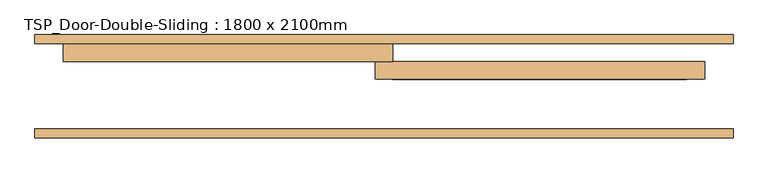
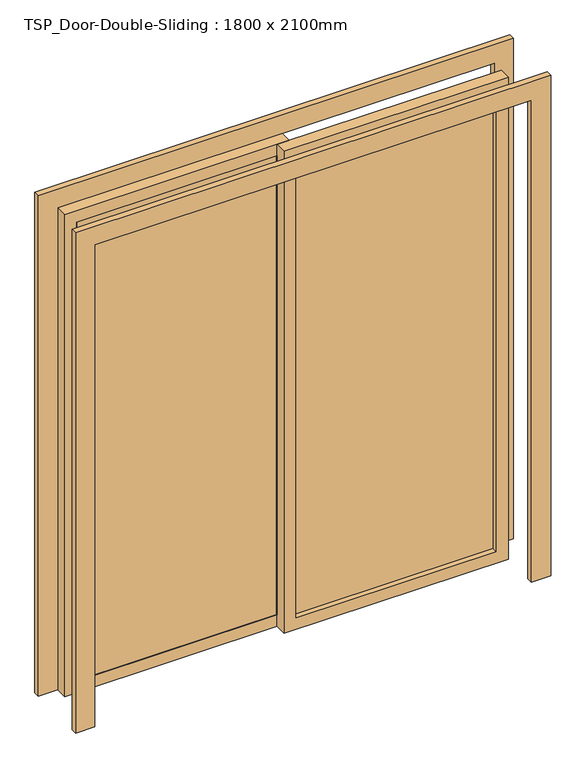
"""IFC4 building model written with IfcOpenShell, lengths in millimetres: door geometry, TSP_Door-Double-Sliding : 1800 x 2100mm."""

from ifc_helpers import new_model, si_unit, frame, origin, place, context, project, spatial, polyline, outline, extrude, source, transform, mapped, element, save


def tsp_door_double_sliding_1800_x_2100mm_5610fb06(model_context):
    return source(origin(), model_context, "Body", "SweptSolid", [
        extrude(outline(polyline([(0.0, 980.0), (2180.0, 980.0), (2180.0, -980.0), (0.0, -980.0), (0.0, -900.0), (2100.0, -900.0), (2100.0, 900.0), (0.0, 900.0), (0.0, 980.0)])), frame((0.0, 247.0, 0.0), z_axis=(0.0, 1.0, 0.0), x_axis=(0.0, 0.0, 1.0)), (0.0, 0.0, 1.0), 25.0),
        extrude(outline(polyline([(0.0, -980.0), (0.0, -900.0), (2100.0, -900.0), (2100.0, 900.0), (0.0, 900.0), (0.0, 980.0), (2180.0, 980.0), (2180.0, -980.0), (0.0, -980.0)])), frame((0.0, -18.0, 0.0), z_axis=(0.0, 1.0, 0.0), x_axis=(0.0, 0.0, 1.0)), (0.0, 0.0, 1.0), 25.0),
        extrude(outline(polyline([(2100.0, 25.0), (2100.0, -900.0), (0.0, -900.0), (0.0, 25.0), (2100.0, 25.0)]), holes=[polyline([(2050.0, -25.0), (50.0, -25.0), (50.0, -850.0), (2050.0, -850.0), (2050.0, -25.0)])]), frame((0.0, 197.0, 0.0), z_axis=(0.0, 1.0, 0.0), x_axis=(0.0, 0.0, 1.0)), (0.0, 0.0, 1.0), 50.0),
        extrude(outline(polyline([(2100.0, -25.0), (0.0, -25.0), (0.0, 900.0), (2100.0, 900.0), (2100.0, -25.0)]), holes=[polyline([(2050.0, 25.0), (2050.0, 850.0), (50.0, 850.0), (50.0, 25.0), (2050.0, 25.0)])]), frame((0.0, 147.0, 0.0), z_axis=(0.0, 1.0, 0.0), x_axis=(0.0, 0.0, 1.0)), (0.0, 0.0, 1.0), 50.0),
        extrude(outline(polyline([(-25.0, 200.025), (-850.0, 200.025), (-850.0, 206.375), (-25.0, 206.375), (-25.0, 200.025)])), frame((0.0, 0.0, 50.0), z_axis=(0.0, 0.0, 1.0), x_axis=(1.0, 0.0, 0.0)), (0.0, 0.0, 1.0), 2000.0),
        extrude(outline(polyline([(25.0, 175.175), (850.0, 175.175), (850.0, 168.825), (25.0, 168.825), (25.0, 175.175)])), frame((0.0, 0.0, 50.0), z_axis=(0.0, 0.0, 1.0), x_axis=(1.0, 0.0, 0.0)), (0.0, 0.0, 1.0), 2000.0),
    ])


if __name__ == "__main__":
    model = new_model("IFC4")
    model_context = context("Model", 3, world=origin())
    ifc_project = project(units=[si_unit("LENGTHUNIT", "METRE", prefix="MILLI")], contexts=[model_context])
    site = spatial("IfcSite", under=ifc_project)
    building = spatial("IfcBuilding", under=site)
    placement = place(None, origin())
    tsp_door_double_sliding_1800_x_2100mm_shape = tsp_door_double_sliding_1800_x_2100mm_5610fb06(model_context)
    element("IfcDoor", 1, ObjectType="TSP_Door-Double-Sliding : 1800 x 2100mm", at=placement, inside=building, context=model_context, shape_type="MappedRepresentation", body=[
        mapped(tsp_door_double_sliding_1800_x_2100mm_shape, transform((0.0, 0.0, 0.0), x_axis=(1.0, 0.0, 0.0), y_axis=(0.0, 1.0, 0.0), z_axis=(0.0, 0.0, 1.0))),
    ])
    save(model, "model.ifc")

# Revit data of these elements
# Type "TSP_Door-Double-Sliding : 1800 x 2100mm"
#   Model = "TSP_DOOR01A"
#   Type Mark = "90"
#   Construction Type Id = "opn-d45"
#   Assembly Code = "C1020"
#   Analytic Construction = "Wood frame, double glass door "
#   Thickness = 50 mm
#   Thermal Resistance (R) = 0.31964 (m²·K)/W
#   Heat Transfer Coefficient (U) = 3.12872 W/(m²·K)
#   Height = 2100 mm
#   Rail Width = 50 mm
#   Stiles = 50 mm
#   Trim Projection Ext = 25 mm
#   Trim Projection Int = 25 mm
#   Trim Width = 80 mm
#   Width = 1800 mm
#   Define Thermal Properties by = 1
#   Glazing = Glass
#   Panel Material = Wood - Birch - Solid Stained Light Low Gloss
#   Trim Material = Paint - Sienna
#   Visual Light Transmittance = 0
#   Solar Heat Gain Coefficient = 0
#   Function = (empty or 0)
#   Wall Closure = (empty or 0)
# Element 1 (IfcDoor, "TSP_Door-Double-Sliding : 1800 x 2100mm")
#   Materials on its faces: "Paint - Sienna", "Wood - Birch - Solid Stained Light Low Gloss", "Glass"
# Materials
#   "Glass": class "Glass", colour RGB 0 128 192, transparency 0.9, Description = "Soda Lime Glass", Cost = 0
#   "Wood - Birch - Solid Stained Light Low Gloss": class "Wood", colour RGB 210 159 95, transparency 0, Cost = 0
#   "Paint - Sienna": class "Miscellaneous", colour RGB 118 70 51, transparency 0, Cost = 0
